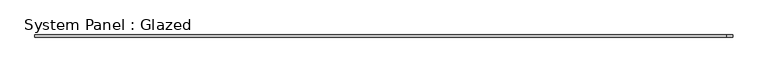
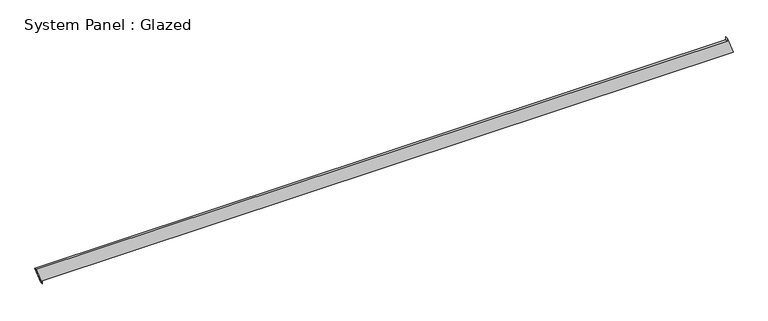
"""IFC4 building model written with IfcOpenShell, lengths in millimetres: plate geometry, System Panel : Glazed."""

from ifc_helpers import new_model, si_unit, frame, origin, place, context, project, spatial, polyline, outline, extrude, source, transform, mapped, element, save


def system_panel_glazed_1e46e190(model_context):
    return source(origin(), model_context, "Body", "SweptSolid", [
        extrude(outline(polyline([(0.0, -3958.6114464), (35.3553391, -3958.6114464), (35.3553391, 4028.3169359), (234.2719876, 3958.4942837), (198.9166485, 3958.4940651), (198.9660296, -4028.3169359), (0.0, -3958.6114464)])), frame((0.0, -49.5, 0.0), z_axis=(0.0, 1.0, 0.0), x_axis=(0.0, 0.0, 1.0)), (0.0, 0.0, 1.0), 25.0),
    ])


if __name__ == "__main__":
    model = new_model("IFC4")
    model_context = context("Model", 3, world=origin())
    ifc_project = project(units=[si_unit("LENGTHUNIT", "METRE", prefix="MILLI")], contexts=[model_context])
    site = spatial("IfcSite", under=ifc_project)
    building = spatial("IfcBuilding", under=site)
    placement = place(None, origin())
    system_panel_glazed_shape = system_panel_glazed_1e46e190(model_context)
    element("IfcPlate", 1, ObjectType="System Panel : Glazed", at=placement, inside=building, context=model_context, shape_type="MappedRepresentation", body=[
        mapped(system_panel_glazed_shape, transform((0.0, 0.0, 0.0), x_axis=(1.0, 0.0, 0.0), y_axis=(0.0, 1.0, 0.0), z_axis=(0.0, 0.0, 1.0))),
    ])
    save(model, "model.ifc")

# Revit data of these elements
# Element 1 (IfcPlate, "System Panel : Glazed")
#   Materials on its faces: "Glass"
# Materials
#   "Glass": class "Glass", colour RGB 218 227 224, transparency 0.85, Description = "Soda Lime Glass", Cost = 0
